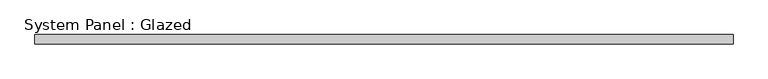
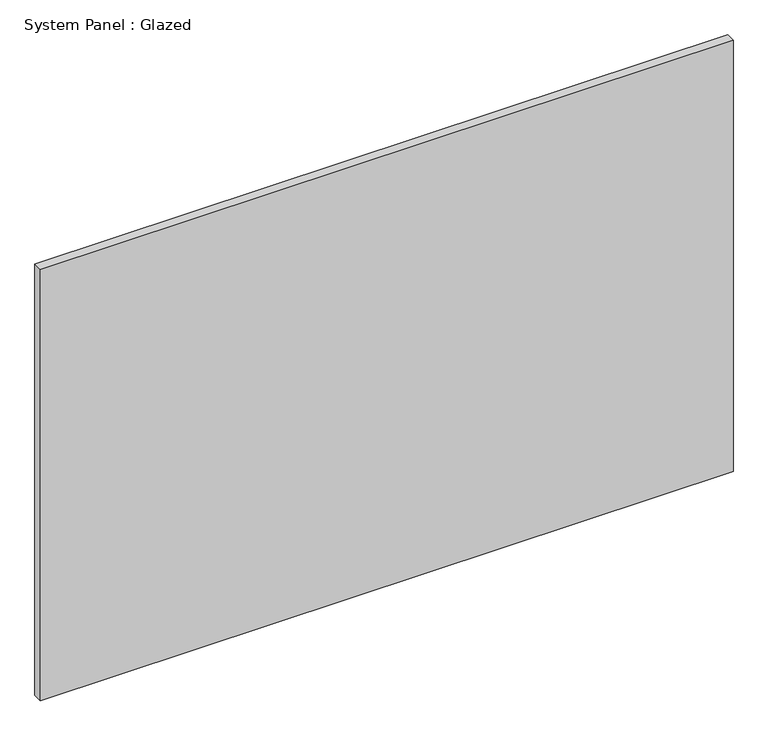
"""IFC4 building model written with IfcOpenShell, lengths in millimetres: plate geometry, System Panel : Glazed."""

from ifc_helpers import new_model, si_unit, origin, origin_with_axes, place, context, project, spatial, polyline, outline, extrude, source, transform, mapped, element, save


def system_panel_glazed_f4bbd109(model_context):
    return source(origin(), model_context, "Body", "SweptSolid", [
        extrude(outline(polyline([(910.8343113, 24.5), (-910.8343113, 24.5), (-910.8343113, 49.5), (910.8343113, 49.5), (910.8343113, 24.5)])), origin_with_axes(), (0.0, 0.0, 1.0), 1200.0),
    ])


if __name__ == "__main__":
    model = new_model("IFC4")
    model_context = context("Model", 3, world=origin())
    ifc_project = project(units=[si_unit("LENGTHUNIT", "METRE", prefix="MILLI")], contexts=[model_context])
    site = spatial("IfcSite", under=ifc_project)
    building = spatial("IfcBuilding", under=site)
    placement = place(None, origin())
    system_panel_glazed_shape = system_panel_glazed_f4bbd109(model_context)
    element("IfcPlate", 1, ObjectType="System Panel : Glazed", at=placement, inside=building, context=model_context, shape_type="MappedRepresentation", body=[
        mapped(system_panel_glazed_shape, transform((0.0, 0.0, 0.0), x_axis=(1.0, 0.0, 0.0), y_axis=(0.0, 1.0, 0.0), z_axis=(0.0, 0.0, 1.0))),
    ])
    save(model, "model.ifc")

# Revit data of these elements
# Element 1 (IfcPlate, "System Panel : Glazed")
#   Materials on its faces: "Glass"
# Materials
#   "Glass": class "Glass", colour RGB 218 227 224, transparency 0.85, Description = "Soda Lime Glass", Cost = 0
